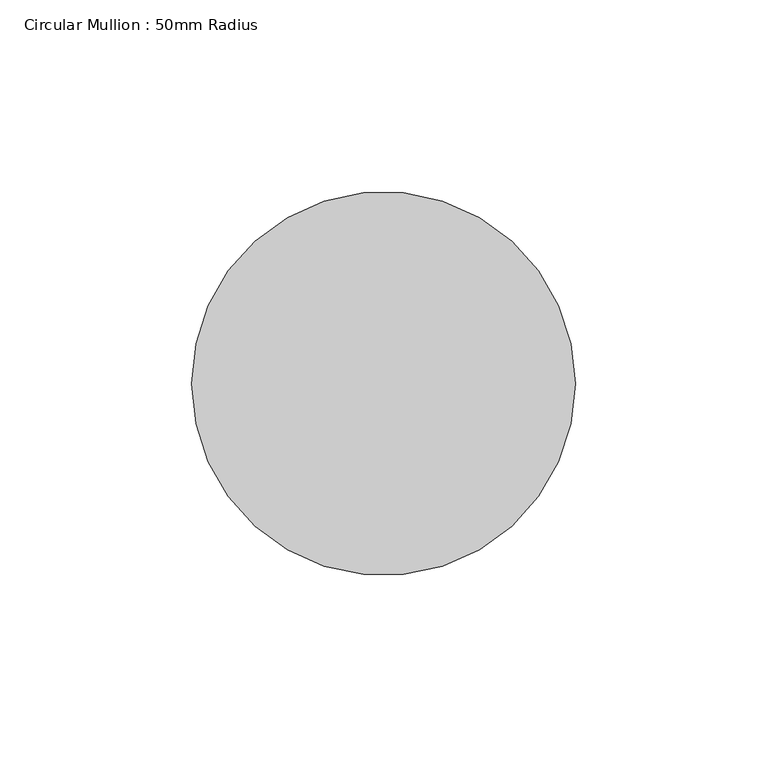
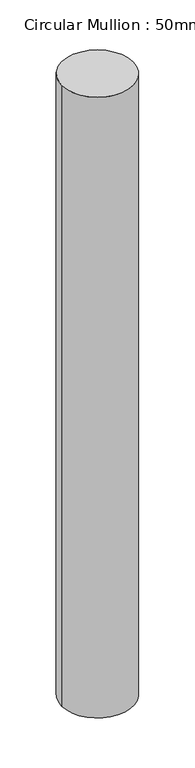
"""IFC4 building model written with IfcOpenShell, lengths in millimetres: member geometry, Circular Mullion : 50mm Radius."""

from ifc_helpers import new_model, si_unit, point, frame, origin, origin_2d, place, context, project, spatial, circle_curve, trimmed, segment, composite_curve, outline, extrude, source, transform, mapped, element, save


def circular_mullion_50mm_radius_adfba775(model_context):
    return source(origin(), model_context, "Body", "SweptSolid", [
        extrude(outline(composite_curve([segment(trimmed(circle_curve(origin_2d(), 50.0), [point((50.0, 0.0))], [point((-50.0, 0.0))], False, "CARTESIAN"), True, "CONTINUOUS"), segment(trimmed(circle_curve(origin_2d(), 50.0), [point((-50.0, 0.0))], [point((50.0, 0.0))], False, "CARTESIAN"), True, "CONTINUOUS")], self_intersect=False)), frame((0.0, 0.0, -917.6793131), z_axis=(0.0, 0.0, 1.0), x_axis=(1.0, 0.0, 0.0)), (0.0, 0.0, 1.0), 917.6793131),
    ])


if __name__ == "__main__":
    model = new_model("IFC4")
    model_context = context("Model", 3, world=origin())
    ifc_project = project(units=[si_unit("LENGTHUNIT", "METRE", prefix="MILLI")], contexts=[model_context])
    site = spatial("IfcSite", under=ifc_project)
    building = spatial("IfcBuilding", under=site)
    placement = place(None, origin())
    circular_mullion_50mm_radius_shape = circular_mullion_50mm_radius_adfba775(model_context)
    element("IfcMember", 1, ObjectType="Circular Mullion : 50mm Radius", at=placement, inside=building, context=model_context, shape_type="MappedRepresentation", body=[
        mapped(circular_mullion_50mm_radius_shape, transform((0.0, 0.0, 0.0), x_axis=(1.0, 0.0, 0.0), y_axis=(0.0, 1.0, 0.0), z_axis=(0.0, 0.0, 1.0))),
    ])
    save(model, "model.ifc")

# Revit data of these elements
# Type "Circular Mullion : 50mm Radius"
#   built-in parameter 1007350 = 0.164042 (stored number, unit not read)
# Element 1 (IfcMember, "Circular Mullion : 50mm Radius")
#   Materials on its faces: "Aluminium"
# Materials
#   "Aluminium": class "Metal", colour RGB 247 247 247, transparency 0, Description = "Aluminium 6061", Cost = 0
